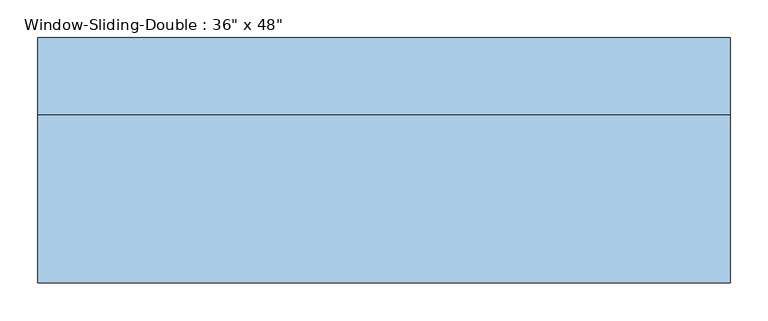
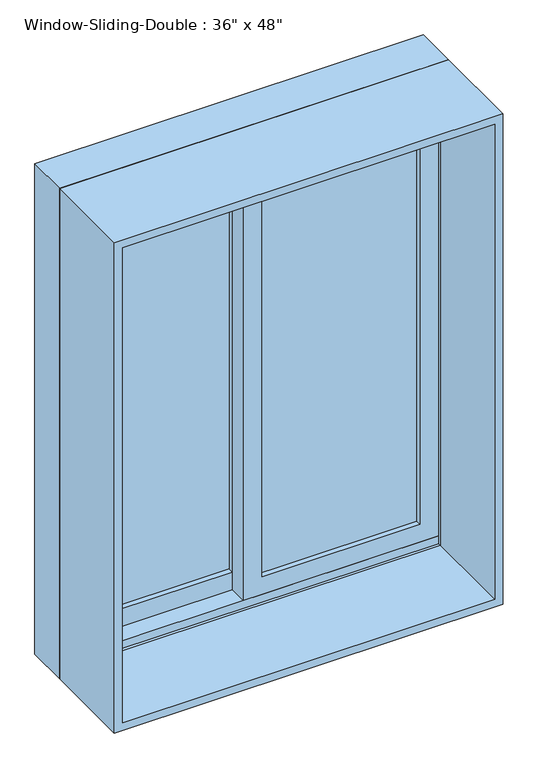
"""IFC4 building model written with IfcOpenShell, lengths in millimetres: window geometry."""

from ifc_helpers import new_model, si_unit, frame, origin, place, context, project, spatial, polyline, outline, extrude, faceted_brep, source, transform, mapped, element, save


def window_690f77e0(model_context):
    return source(origin(), model_context, "Body", "SolidModel", [
        faceted_brep([(-457.2, 66.04, 914.4), (-457.2, 167.64, 914.4), (457.2, 167.64, 914.4), (457.2, 66.04, 914.4), (-416.2778905, 167.64, 2092.6778905), (-416.2778905, 161.29, 2092.6778905), (-416.2778905, 161.29, 933.45), (-416.2778905, 167.64, 933.45), (416.2778905, 161.29, 2092.6778905), (416.2778905, 161.29, 933.45), (438.15, 161.29, 933.45), (438.15, 161.29, 2114.55), (-438.15, 161.29, 2114.55), (-438.15, 161.29, 933.45), (-438.15, 66.04, 2114.55), (-438.15, 66.04, 933.45), (-438.15, 72.39, 933.45), (-438.15, 72.39, 952.5), (-438.15, 116.84, 952.5), (-438.15, 116.84, 933.45), (457.2, 66.04, 2133.6), (-457.2, 66.04, 2133.6), (438.15, 66.04, 2114.55), (438.15, 66.04, 933.45), (-457.2, 167.64, 2133.6), (457.2, 167.64, 2133.6), (416.2778905, 167.64, 933.45), (416.2778905, 167.64, 2092.6778905), (438.15, 116.84, 933.45), (438.15, 116.84, 952.5), (438.15, 72.39, 952.5), (438.15, 72.39, 933.45)], [[[0, 1, 2, 3]], [[4, 5, 6, 7]], [[5, 8, 9, 10, 11, 12, 13, 6]], [[12, 14, 15, 16, 17, 18, 19, 13]], [[0, 3, 20, 21], [22, 23, 15, 14]], [[24, 1, 0, 21]], [[2, 1, 24, 25], [4, 7, 26, 27]], [[5, 4, 27, 8]], [[12, 11, 22, 14]], [[21, 20, 25, 24]], [[8, 27, 26, 9]], [[22, 11, 10, 28, 29, 30, 31, 23]], [[20, 3, 2, 25]], [[26, 7, 6, 13, 19, 28, 10, 9]], [[28, 19, 18, 29]], [[29, 18, 17, 30]], [[30, 17, 16, 31]], [[15, 23, 31, 16]]]),
        extrude(outline(polyline([(2133.6, -457.2), (914.4, -457.2), (914.4, 457.2), (2133.6, 457.2), (2133.6, -457.2)]), holes=[polyline([(2114.55, 438.15), (933.45, 438.15), (933.45, -438.15), (2114.55, -438.15), (2114.55, 438.15)])]), frame((0.0, -156.21, 0.0), z_axis=(0.0, 1.0, 0.0), x_axis=(0.0, 0.0, 1.0)), (0.0, 0.0, 1.0), 222.25),
        extrude(outline(polyline([(393.7, 104.14), (393.7, 97.79), (22.225, 97.79), (22.225, 104.14), (393.7, 104.14)])), frame((0.0, 0.0, 996.95), z_axis=(0.0, 0.0, 1.0), x_axis=(1.0, 0.0, 0.0)), (0.0, 0.0, 1.0), 1073.15),
        extrude(outline(polyline([(393.7, 91.44), (393.7, 85.09), (22.225, 85.09), (22.225, 91.44), (393.7, 91.44)])), frame((0.0, 0.0, 996.95), z_axis=(0.0, 0.0, 1.0), x_axis=(1.0, 0.0, 0.0)), (0.0, 0.0, 1.0), 1073.15),
        extrude(outline(polyline([(-22.225, 148.59), (-22.225, 142.24), (-393.7, 142.24), (-393.7, 148.59), (-22.225, 148.59)])), frame((0.0, 0.0, 996.95), z_axis=(0.0, 0.0, 1.0), x_axis=(1.0, 0.0, 0.0)), (0.0, 0.0, 1.0), 1073.15),
        extrude(outline(polyline([(-22.225, 135.89), (-22.225, 129.54), (-393.7, 129.54), (-393.7, 135.89), (-22.225, 135.89)])), frame((0.0, 0.0, 996.95), z_axis=(0.0, 0.0, 1.0), x_axis=(1.0, 0.0, 0.0)), (0.0, 0.0, 1.0), 1073.15),
        extrude(outline(polyline([(933.45, -438.15), (933.45, 22.225), (2114.55, 22.225), (2114.55, -438.15), (933.45, -438.15)]), holes=[polyline([(2070.1, -22.225), (996.95, -22.225), (996.95, -393.7), (2070.1, -393.7), (2070.1, -22.225)])]), frame((0.0, 116.84, 0.0), z_axis=(0.0, 1.0, 0.0), x_axis=(0.0, 0.0, 1.0)), (0.0, 0.0, 1.0), 44.45),
        extrude(outline(polyline([(952.5, 438.15), (2114.55, 438.15), (2114.55, -22.225), (952.5, -22.225), (952.5, 438.15)]), holes=[polyline([(996.95, 22.225), (2070.1, 22.225), (2070.1, 393.7), (996.95, 393.7), (996.95, 22.225)])]), frame((0.0, 72.39, 0.0), z_axis=(0.0, 1.0, 0.0), x_axis=(0.0, 0.0, 1.0)), (0.0, 0.0, 1.0), 44.45),
    ])


if __name__ == "__main__":
    model = new_model("IFC4")
    model_context = context("Model", 3, world=origin())
    ifc_project = project(units=[si_unit("LENGTHUNIT", "METRE", prefix="MILLI")], contexts=[model_context])
    site = spatial("IfcSite", under=ifc_project)
    building = spatial("IfcBuilding", under=site)
    placement = place(None, origin())
    window_shape = window_690f77e0(model_context)
    element("IfcWindow", 1, ObjectType="Window-Sliding-Double : 36\" x 48\"", at=placement, inside=building, context=model_context, shape_type="MappedRepresentation", body=[
        mapped(window_shape, transform((0.0, 0.0, 0.0), x_axis=(1.0, 0.0, 0.0), y_axis=(0.0, 1.0, 0.0), z_axis=(0.0, 0.0, 1.0))),
    ])
    save(model, "model.ifc")

# Revit data of these elements
# Type "Window-Sliding-Double : 36\" x 48\""
#   Type Mark = "E"
#   Fire Rating = "0.5h"
#   Assembly Code = "B2020100"
#   Analytic Construction = "Double glazing - domestic"
#   Window Inset [instance default] = 0' - 0"
#   Wall Thickness [instance default] = 0' - 6"
#   Visual Light Transmittance = 0.81
#   Thermal Resistance (R) = 1.8146 (h·ft²·°F)/BTU
#   Solar Heat Gain Coefficient = 0.76
#   Muntin Width = 1' - 2 5/8"
#   Muntin Height = 3' - 6 1/4"
#   Interior Wall Closure [instance default] = 0' - 2 3/4"
#   Heat Transfer Coefficient (U) = 0.5511 BTU/(h·ft²·°F)
#   Frame Extension [instance default] = 0' - 0 1/4"
#   Exterior Wall Closure [instance default] = 0' - 1 1/4"
#   Rough Width = 3' - 0 1/2"
#   Rough Height = 4' - 0 1/2"
#   Height = 4' - 0"
#   Extension Jamb [instance default] = 0' - 2 3/4"
#   Default Sill Height = 3' - 0"
#   Width = 3' - 0"
#   Interior Trim Visibility [instance default] = yes
#   Indicator Visibility [instance default] = yes
#   Exterior Trim Visibility [instance default] = yes
#   Muntin Visibility = yes
#   Extension Jamb Visibility [instance default] = yes
#   Muntin Pattern = Muntin Pattern_2x2 : Muntin Pattern_2x2
#   Interior Trim Material = Wood - Stained
#   Interior Trim = Trim-Window-Interior-Flat : Picture Frame
#   Interior Frame Material = Wood - Stained
#   Glass Panel Material = Glass
#   Exterior Trim Material = Clad - White
#   Exterior Trim = Trim-Window-Exterior-Flat : with Sill
#   Exterior Frame Material = Clad - White
#   Wall Closure = (empty or 0)
# Element 1 (IfcWindow, "Window-Sliding-Double : 36\" x 48\"")
#   Wall Thickness = 1' - 0"
#   Extension Jamb = 0' - 8 3/4"
#   Materials on its faces: "Wood - Stained", "Glass", "Clad - White"
# Materials
#   "Wood - Stained": class "Wood", colour RGB 224 178 126, transparency 0, Cost = 0
#   "Glass": class "Unassigned", colour RGB 0 128 192, transparency 0.75, Description = "Glass"
#   "Clad - White": class "Wood", colour RGB 242 242 238, transparency 0, Cost = 0
